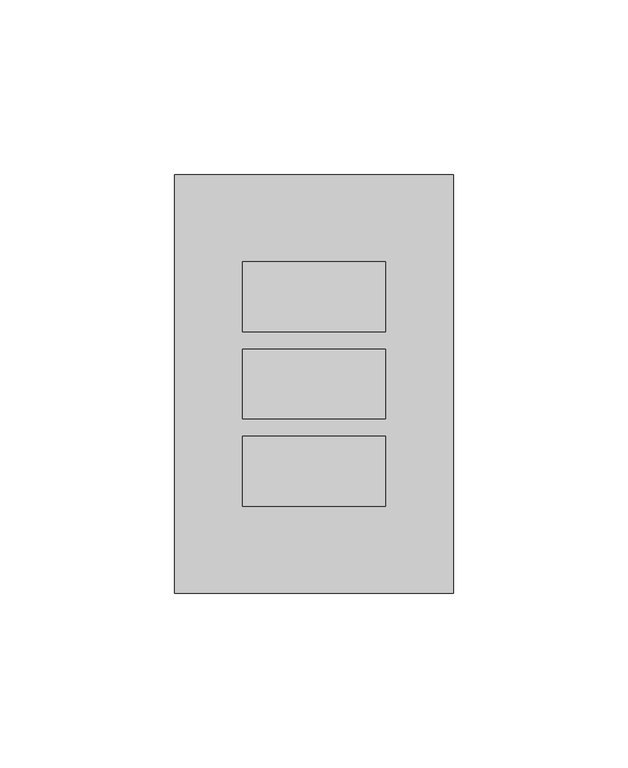
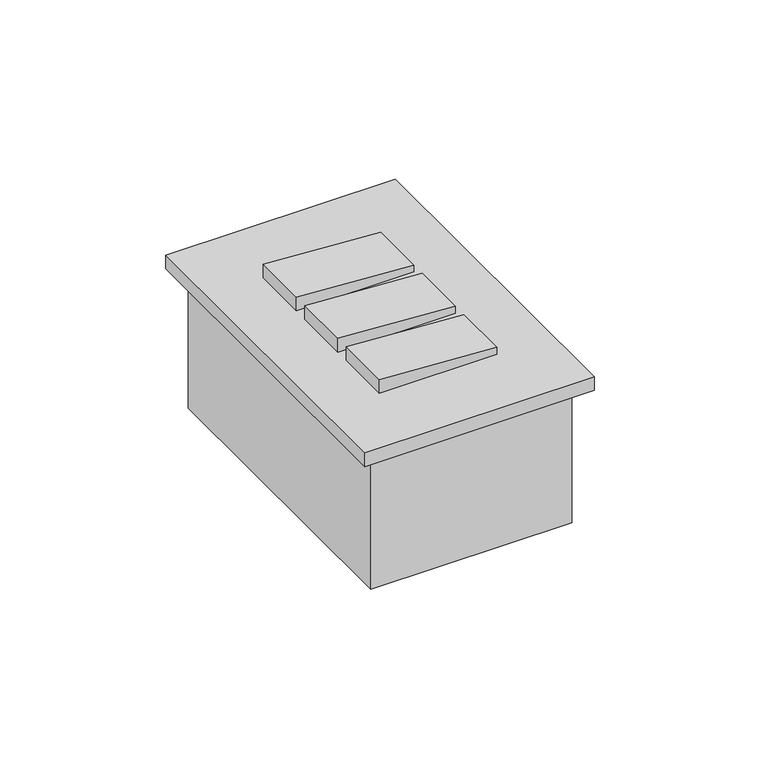
"""IFC4 building model written with IfcOpenShell, lengths in millimetres: proxy geometry, CAIXA VERTICE V7 : Interruptor 3s."""

import ifcopenshell
import ifcopenshell.guid

model = None  # the IFC model being written
_history = None  # IfcOwnerHistory: only IFC2X3 demands one
_inside = {}  # id of a spatial element -> (the spatial element, [elements in it])
_under = {}  # id of a project, library or spatial element -> (it, [spatial elements below it])
_declared = {}  # id of a project -> (the project, [libraries it declares])
_typed = {}  # id of a type object -> (the type object, [elements of that type])
_made_of = {}  # id of a material, layer set ... -> (it, [elements and type objects made of it])


def new_model(schema):
    """Start an empty IFC model of exactly this schema.

    Asked for "IFC4X3", IfcOpenShell would pick the latest addendum, in which some entities
    have other attributes; the version numbers below select the first issue.
    IFC2X3 requires an IfcOwnerHistory on every rooted entity: one is made here for all.
    """
    global model, _history
    if schema == "IFC4X3":
        model = ifcopenshell.file(schema_version=(4, 3, 0, 0))
    else:
        model = ifcopenshell.file(schema=schema)
    _inside.clear()
    _under.clear()
    _declared.clear()
    _typed.clear()
    _made_of.clear()
    _history = None
    if model.schema == "IFC2X3":
        org = make("IfcOrganization", Name="unknown")
        user = make(
            "IfcPersonAndOrganization",
            ThePerson=make("IfcPerson", FamilyName="unknown"),
            TheOrganization=org,
        )
        app = make(
            "IfcApplication",
            ApplicationDeveloper=org,
            Version="unknown",
            ApplicationFullName="unknown",
            ApplicationIdentifier="unknown",
        )
        _history = make(
            "IfcOwnerHistory",
            OwningUser=user,
            OwningApplication=app,
            ChangeAction="ADDED",
            CreationDate=0,
        )
    return model


def make(cls, **values):
    """One entity of the class cls with the attributes given. An attribute that is None is left unset."""
    return model.create_entity(
        cls, **{name: value for name, value in values.items() if value is not None}
    )


def rooted(cls, **values):
    """An entity with a GlobalId (a new one), such as an element, a storey or a relation."""
    return make(cls, GlobalId=ifcopenshell.guid.new(), OwnerHistory=_history, **values)


def si_unit(unit_type, name, prefix=None):
    """IfcSIUnit, for example si_unit("LENGTHUNIT", "METRE", prefix="MILLI")."""
    return make("IfcSIUnit", UnitType=unit_type, Prefix=prefix, Name=name)


def assignment(units):
    """IfcUnitAssignment: the units of a project."""
    return None if units is None else make("IfcUnitAssignment", Units=units)


def point(xyz):
    """IfcCartesianPoint."""
    return None if xyz is None else make("IfcCartesianPoint", Coordinates=xyz)


def direction(xyz):
    """IfcDirection."""
    return None if xyz is None else make("IfcDirection", DirectionRatios=xyz)


def frame(location, z_axis=None, x_axis=None):
    """IfcAxis2Placement3D, a coordinate frame: its origin and axes. An axis left out is left unset."""
    return make(
        "IfcAxis2Placement3D",
        Location=point(location),
        Axis=direction(z_axis),
        RefDirection=direction(x_axis),
    )


def origin():
    """The frame at (0, 0, 0) with its axes left unset."""
    return frame((0.0, 0.0, 0.0))


def origin_with_axes():
    """The frame at (0, 0, 0) with the z axis (0, 0, 1) and the x axis (1, 0, 0) written out."""
    return frame((0.0, 0.0, 0.0), z_axis=(0.0, 0.0, 1.0), x_axis=(1.0, 0.0, 0.0))


def place(relative_to, where):
    """IfcLocalPlacement: puts the frame where relative to a parent placement (None: the world)."""
    return make(
        "IfcLocalPlacement", PlacementRelTo=relative_to, RelativePlacement=where
    )


def context(
    kind, dimensions, precision=None, world=None, true_north=None, identifier=None
):
    """IfcGeometricRepresentationContext, for example the 3D "Model" context."""
    return make(
        "IfcGeometricRepresentationContext",
        ContextIdentifier=identifier,
        ContextType=kind,
        CoordinateSpaceDimension=dimensions,
        Precision=precision,
        WorldCoordinateSystem=world,
        TrueNorth=true_north,
    )


def project(units=None, contexts=None):
    """IfcProject with its units and contexts."""
    return rooted(
        "IfcProject",
        Name="project",
        RepresentationContexts=contexts,
        UnitsInContext=assignment(units),
    )


def spatial(cls, under=None, at=None, **own):
    """A site, building, storey or space (cls), placed at a placement, below another one or the project."""
    s = rooted(cls, ObjectPlacement=at, **own)
    if under is not None:
        _under.setdefault(under.id(), (under, []))[1].append(s)
    return s


def polyline(points):
    """IfcPolyline through the points."""
    return make("IfcPolyline", Points=[point(p) for p in points])


def outline(outer, holes=None, kind="AREA"):
    """IfcArbitraryClosedProfileDef: a profile drawn as a closed curve; with holes, ...WithVoids."""
    if holes is None:
        return make("IfcArbitraryClosedProfileDef", ProfileType=kind, OuterCurve=outer)
    return make(
        "IfcArbitraryProfileDefWithVoids",
        ProfileType=kind,
        OuterCurve=outer,
        InnerCurves=holes,
    )


def extrude(swept, where, along, depth):
    """IfcExtrudedAreaSolid: the profile swept, set in the frame where, extruded along a direction by depth."""
    return make(
        "IfcExtrudedAreaSolid",
        SweptArea=swept,
        Position=where,
        ExtrudedDirection=direction(along),
        Depth=depth,
    )


def faces_of(points, faces, orient=None, outer=None):
    """IfcFace entities. A face is a list of loops; a loop is a list of indices into points, from 0.

    orient and outer hold one flag for each loop. By default every Orientation is true, the
    first loop of a face is its IfcFaceOuterBound and the others are IfcFaceBound.
    """
    made = []
    for i, loops in enumerate(faces):
        bounds = []
        for j, loop in enumerate(loops):
            is_outer = j == 0 if outer is None else outer[i][j]
            bounds.append(
                make(
                    "IfcFaceOuterBound" if is_outer else "IfcFaceBound",
                    Bound=make("IfcPolyLoop", Polygon=[points[k] for k in loop]),
                    Orientation=True if orient is None else orient[i][j],
                )
            )
        made.append(make("IfcFace", Bounds=bounds))
    return made


def faceted_brep(points, faces, orient=None, outer=None, voids=None):
    """IfcFacetedBrep: a solid bounded by flat faces; with voids (closed shells), ...WithVoids."""
    shared = [point(p) for p in points]
    hull = make("IfcClosedShell", CfsFaces=faces_of(shared, faces, orient, outer))
    if voids is None:
        return make("IfcFacetedBrep", Outer=hull)
    return make(
        "IfcFacetedBrepWithVoids",
        Outer=hull,
        Voids=[
            make(cls, CfsFaces=faces_of(shared, fs, o, b)) for cls, fs, o, b in voids
        ],
    )


def shape(context_of_items, identifier, shape_type, items):
    """IfcShapeRepresentation: the items that make up one representation, for example the "Body"."""
    return make(
        "IfcShapeRepresentation",
        ContextOfItems=context_of_items,
        RepresentationIdentifier=identifier,
        RepresentationType=shape_type,
        Items=items,
    )


def source(mapping_origin, context_of_items, identifier, shape_type, items):
    """IfcRepresentationMap: a shape defined once, which mapped items show again and again."""
    return make(
        "IfcRepresentationMap",
        MappingOrigin=mapping_origin,
        MappedRepresentation=shape(context_of_items, identifier, shape_type, items),
    )


def transform(
    local_origin,
    x_axis=None,
    y_axis=None,
    z_axis=None,
    scale=None,
    scale2=None,
    scale3=None,
    uniform=True,
):
    """IfcCartesianTransformationOperator3D, or its non-uniform kind. x_axis, y_axis, z_axis: its Axis1, 2, 3."""
    if uniform:
        return make(
            "IfcCartesianTransformationOperator3D",
            Axis1=direction(x_axis),
            Axis2=direction(y_axis),
            LocalOrigin=point(local_origin),
            Scale=scale,
            Axis3=direction(z_axis),
        )
    return make(
        "IfcCartesianTransformationOperator3DnonUniform",
        Axis1=direction(x_axis),
        Axis2=direction(y_axis),
        LocalOrigin=point(local_origin),
        Scale=scale,
        Axis3=direction(z_axis),
        Scale2=scale2,
        Scale3=scale3,
    )


def mapped(mapping_source, mapping_target):
    """IfcMappedItem: shows the shape of a source again, moved by a transform."""
    return make(
        "IfcMappedItem", MappingSource=mapping_source, MappingTarget=mapping_target
    )


def made_of(thing, what):
    """Note that an element or type object is made of a material, layer set ...; save() writes the relation."""
    if what is not None:
        _made_of.setdefault(what.id(), (what, []))[1].append(thing)
    return thing


def element(
    cls,
    number,
    at=None,
    inside=None,
    cuts=None,
    type_object=None,
    material=None,
    context=None,
    identifier="Body",
    shape_type=None,
    held_by="IfcProductDefinitionShape",
    body=None,
    shapes=None,
    **own,
):
    """One element of the class cls, such as IfcWall. Its Tag is "e" and its number.

    at: its placement. inside: the storey or other place that contains it. cuts: it is an
    opening in that element (IfcRelVoidsElement). A single representation is given by context,
    identifier, shape_type and body (its items); several are given by shapes. held_by: the class
    of the entity that holds the representations. save() writes the other relations.
    """
    e = rooted(cls, Tag="e%d" % number, ObjectPlacement=at, **own)
    if body is not None:
        shapes = [shape(context, identifier, shape_type, body)]
    if shapes is not None:
        e.Representation = make(held_by, Representations=shapes)
    if inside is not None:
        _inside.setdefault(inside.id(), (inside, []))[1].append(e)
    if cuts is not None:
        rooted(
            "IfcRelVoidsElement", RelatingBuildingElement=cuts, RelatedOpeningElement=e
        )
    if type_object is not None:
        _typed.setdefault(type_object.id(), (type_object, []))[1].append(e)
    return made_of(e, material)


def aggregate(whole, parts):
    """IfcRelAggregates: a whole, such as a stair, and the parts it consists of."""
    return rooted("IfcRelAggregates", RelatingObject=whole, RelatedObjects=parts)


def save(model, path):
    """Write the relations noted so far, then the file.

    IfcRelAggregates (storeys below a building ...), IfcRelContainedInSpatialStructure (elements
    in a storey), IfcRelDefinesByType, IfcRelAssociatesMaterial and IfcRelDeclares: one each for
    every whole, place, type object, material and project.
    """
    for whole, parts in _under.values():
        aggregate(whole, parts)
    for where, things in _inside.values():
        rooted(
            "IfcRelContainedInSpatialStructure",
            RelatedElements=things,
            RelatingStructure=where,
        )
    for kind, things in _typed.values():
        rooted("IfcRelDefinesByType", RelatedObjects=things, RelatingType=kind)
    for what, things in _made_of.values():
        rooted("IfcRelAssociatesMaterial", RelatedObjects=things, RelatingMaterial=what)
    for by, libraries in _declared.values():
        rooted("IfcRelDeclares", RelatingContext=by, RelatedDefinitions=libraries)
    model.write(path)


def electrical_fixtures_58d60563(model_context):
    return source(origin(), model_context, "Body", "SolidModel", [
        extrude(outline(polyline([(5.0, 20.5), (7.5, 20.5), (10.0, -20.5), (5.0, -20.5), (5.0, 20.5)])), frame((0.0, -1085.0, 0.0), z_axis=(0.0, 1.0, 0.0), x_axis=(0.0, 0.0, 1.0)), (0.0, 0.0, 1.0), 20.0),
        extrude(outline(polyline([(5.0, 20.5), (7.5, 20.5), (10.0, -20.5), (5.0, -20.5), (5.0, 20.5)])), frame((0.0, -1110.0, 0.0), z_axis=(0.0, 1.0, 0.0), x_axis=(0.0, 0.0, 1.0)), (0.0, 0.0, 1.0), 20.0),
        extrude(outline(polyline([(5.0, 20.5), (7.5, 20.5), (10.0, -20.5), (5.0, -20.5), (5.0, 20.5)])), frame((0.0, -1135.0, 0.0), z_axis=(0.0, 1.0, 0.0), x_axis=(0.0, 0.0, 1.0)), (0.0, 0.0, 1.0), 20.0),
        faceted_brep([(33.0, -1047.0, -48.0), (-33.0, -1047.0, -48.0), (-33.0, -1153.0, -48.0), (33.0, -1153.0, -48.0), (35.0, -1155.0, -50.0), (-35.0, -1155.0, -50.0), (-35.0, -1045.0, -50.0), (35.0, -1045.0, -50.0), (35.0, -1155.0, 0.0), (-35.0, -1155.0, 0.0), (-35.0, -1045.0, 0.0), (35.0, -1045.0, 0.0), (33.0, -1153.0, 0.0), (-33.0, -1153.0, 0.0), (-33.0, -1047.0, 0.0), (33.0, -1047.0, 0.0)], [[[0, 1, 2, 3]], [[4, 5, 6, 7]], [[4, 8, 9, 5]], [[9, 10, 6, 5]], [[10, 11, 7, 6]], [[11, 8, 4, 7]], [[8, 11, 10, 9], [12, 13, 14, 15]], [[15, 0, 3, 12]], [[14, 1, 0, 15]], [[13, 2, 1, 14]], [[12, 3, 2, 13]]]),
        extrude(outline(polyline([(40.0, -1160.0), (-40.0, -1160.0), (-40.0, -1040.0), (40.0, -1040.0), (40.0, -1160.0)])), origin_with_axes(), (0.0, 0.0, 1.0), 5.0),
    ])


if __name__ == "__main__":
    model = new_model("IFC4")
    model_context = context("Model", 3, world=origin())
    ifc_project = project(units=[si_unit("LENGTHUNIT", "METRE", prefix="MILLI")], contexts=[model_context])
    site = spatial("IfcSite", under=ifc_project)
    building = spatial("IfcBuilding", under=site)
    placement = place(None, origin())
    electrical_fixtures_shape = electrical_fixtures_58d60563(model_context)
    element("IfcBuildingElementProxy", 1, Name="CAIXA VERTICE V7 : Interruptor 3s", ObjectType="CAIXA VERTICE V7 : Interruptor 3s", at=placement, inside=building, context=model_context, shape_type="MappedRepresentation", body=[
        mapped(electrical_fixtures_shape, transform((0.0, 0.0, 0.0), x_axis=(1.0, 0.0, 0.0), y_axis=(0.0, 1.0, 0.0), z_axis=(0.0, 0.0, 1.0))),
    ])
    save(model, "model.ifc")

# Revit data of these elements
# Type "CAIXA VERTICE V7 : Interruptor 3s"
#   URL = "www.facebook.com/verticetreinamentos"
#   SEÇÃO [instance default] = ""
#   Rotação [instance default] = 0.00°
#   LARGURA DA TAMPA = 0.08 m
#   BORDA = 0.01 m
#   ALTURA DE INSTALAÇÃO [instance default] = 1.10 m
#   Distância Anotação [instance default] = 0.0015 m
#   ALTURA DA TAMPA = 0.12 m
#   Vertical [instance default] = yes
#   VER SEÇÃO [instance default] = yes
#   SHADE ESQ [instance default] = no
#   SHADE DIR [instance default] = yes
#   HORIZONTAL [instance default] = no
#   ANDAR COM A LEGENDA [instance default] = 0
#   Material Tampa [instance default] = Plástico, branco opaco
#   Caixa = element 1798511
#   Anotação = element 1798523
#   Default Elevation = 0
# Element 1 (IfcBuildingElementProxy, "CAIXA VERTICE V7 : Interruptor 3s")
#   SEÇÃO = "3"
#   Distância Anotação = 0.0035 m
#   ANDAR COM A LEGENDA = 1
#   Materials on its faces: "Plástico, branco opaco"
# Materials
#   "Plástico, branco opaco": class "Plástico", colour RGB 120 120 120, transparency 0, Description = "Plastic, generic, opaque white", Cost = 0
